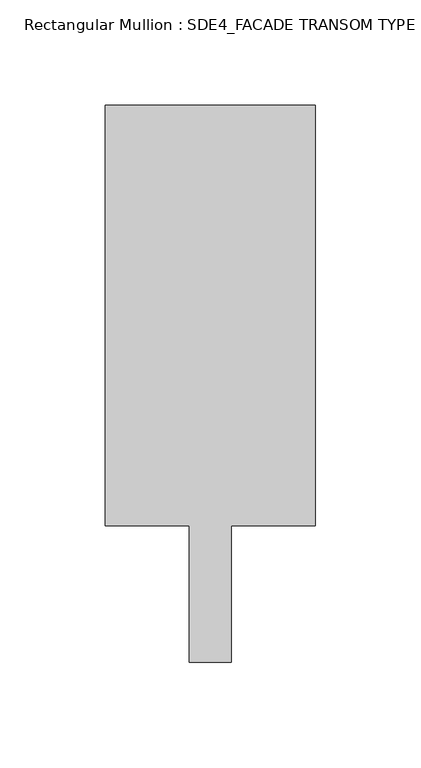
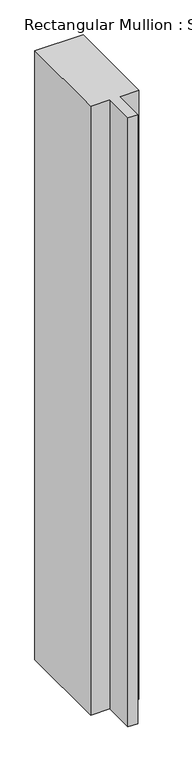
"""IFC4 building model written with IfcOpenShell, lengths in millimetres: member geometry, Rectangular Mullion : SDE4_FACADE TRANSOM TYPE 2."""

from ifc_helpers import new_model, si_unit, frame, origin, place, context, project, spatial, polyline, outline, extrude, source, transform, mapped, element, save


def rectangular_mullion_sde4_facade_transom_type_2_26d4236c(model_context):
    return source(origin(), model_context, "Body", "SweptSolid", [
        extrude(outline(polyline([(50.0, 132.5), (50.0, -67.5), (10.0, -67.5), (10.0, -132.5), (-10.0, -132.5), (-10.0, -67.5), (-50.0, -67.5), (-50.0, 132.5), (50.0, 132.5)])), frame((0.0, 0.0, -1335.0), z_axis=(0.0, 0.0, 1.0), x_axis=(1.0, 0.0, 0.0)), (0.0, 0.0, 1.0), 1335.0),
    ])


if __name__ == "__main__":
    model = new_model("IFC4")
    model_context = context("Model", 3, world=origin())
    ifc_project = project(units=[si_unit("LENGTHUNIT", "METRE", prefix="MILLI")], contexts=[model_context])
    site = spatial("IfcSite", under=ifc_project)
    building = spatial("IfcBuilding", under=site)
    placement = place(None, origin())
    rectangular_mullion_sde4_facade_transom_type_2_shape = rectangular_mullion_sde4_facade_transom_type_2_26d4236c(model_context)
    element("IfcMember", 1, ObjectType="Rectangular Mullion : SDE4_FACADE TRANSOM TYPE 2", at=placement, inside=building, context=model_context, shape_type="MappedRepresentation", body=[
        mapped(rectangular_mullion_sde4_facade_transom_type_2_shape, transform((0.0, 0.0, 0.0), x_axis=(1.0, 0.0, 0.0), y_axis=(0.0, 1.0, 0.0), z_axis=(0.0, 0.0, 1.0))),
    ])
    save(model, "model.ifc")

# Revit data of these elements
# Type "Rectangular Mullion : SDE4_FACADE TRANSOM TYPE 2"
#   built-in parameter 1007322 = 0.869423 (stored number, unit not read)
#   built-in parameter 1007321 = 0.164042 (stored number, unit not read)
#   built-in parameter 1007320 = 0.164042 (stored number, unit not read)
